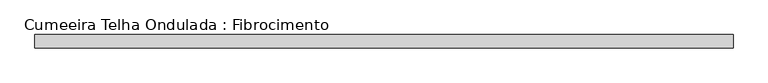
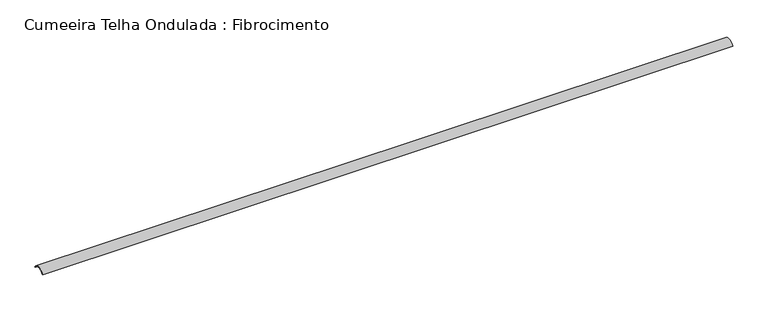
"""IFC4 building model written with IfcOpenShell, lengths in millimetres: beam geometry, Cumeeira Telha Ondulada : Fibrocimento."""

import ifcopenshell
import ifcopenshell.guid

model = None  # the IFC model being written
_history = None  # IfcOwnerHistory: only IFC2X3 demands one
_inside = {}  # id of a spatial element -> (the spatial element, [elements in it])
_under = {}  # id of a project, library or spatial element -> (it, [spatial elements below it])
_declared = {}  # id of a project -> (the project, [libraries it declares])
_typed = {}  # id of a type object -> (the type object, [elements of that type])
_made_of = {}  # id of a material, layer set ... -> (it, [elements and type objects made of it])


def new_model(schema):
    """Start an empty IFC model of exactly this schema.

    Asked for "IFC4X3", IfcOpenShell would pick the latest addendum, in which some entities
    have other attributes; the version numbers below select the first issue.
    IFC2X3 requires an IfcOwnerHistory on every rooted entity: one is made here for all.
    """
    global model, _history
    if schema == "IFC4X3":
        model = ifcopenshell.file(schema_version=(4, 3, 0, 0))
    else:
        model = ifcopenshell.file(schema=schema)
    _inside.clear()
    _under.clear()
    _declared.clear()
    _typed.clear()
    _made_of.clear()
    _history = None
    if model.schema == "IFC2X3":
        org = make("IfcOrganization", Name="unknown")
        user = make(
            "IfcPersonAndOrganization",
            ThePerson=make("IfcPerson", FamilyName="unknown"),
            TheOrganization=org,
        )
        app = make(
            "IfcApplication",
            ApplicationDeveloper=org,
            Version="unknown",
            ApplicationFullName="unknown",
            ApplicationIdentifier="unknown",
        )
        _history = make(
            "IfcOwnerHistory",
            OwningUser=user,
            OwningApplication=app,
            ChangeAction="ADDED",
            CreationDate=0,
        )
    return model


def make(cls, **values):
    """One entity of the class cls with the attributes given. An attribute that is None is left unset."""
    return model.create_entity(
        cls, **{name: value for name, value in values.items() if value is not None}
    )


def rooted(cls, **values):
    """An entity with a GlobalId (a new one), such as an element, a storey or a relation."""
    return make(cls, GlobalId=ifcopenshell.guid.new(), OwnerHistory=_history, **values)


def si_unit(unit_type, name, prefix=None):
    """IfcSIUnit, for example si_unit("LENGTHUNIT", "METRE", prefix="MILLI")."""
    return make("IfcSIUnit", UnitType=unit_type, Prefix=prefix, Name=name)


def assignment(units):
    """IfcUnitAssignment: the units of a project."""
    return None if units is None else make("IfcUnitAssignment", Units=units)


def point(xyz):
    """IfcCartesianPoint."""
    return None if xyz is None else make("IfcCartesianPoint", Coordinates=xyz)


def direction(xyz):
    """IfcDirection."""
    return None if xyz is None else make("IfcDirection", DirectionRatios=xyz)


def frame(location, z_axis=None, x_axis=None):
    """IfcAxis2Placement3D, a coordinate frame: its origin and axes. An axis left out is left unset."""
    return make(
        "IfcAxis2Placement3D",
        Location=point(location),
        Axis=direction(z_axis),
        RefDirection=direction(x_axis),
    )


def frame_2d(location, x_axis=None):
    """IfcAxis2Placement2D, a coordinate frame in the plane: its origin and x axis."""
    return make(
        "IfcAxis2Placement2D", Location=point(location), RefDirection=direction(x_axis)
    )


def origin():
    """The frame at (0, 0, 0) with its axes left unset."""
    return frame((0.0, 0.0, 0.0))


def place(relative_to, where):
    """IfcLocalPlacement: puts the frame where relative to a parent placement (None: the world)."""
    return make(
        "IfcLocalPlacement", PlacementRelTo=relative_to, RelativePlacement=where
    )


def context(
    kind, dimensions, precision=None, world=None, true_north=None, identifier=None
):
    """IfcGeometricRepresentationContext, for example the 3D "Model" context."""
    return make(
        "IfcGeometricRepresentationContext",
        ContextIdentifier=identifier,
        ContextType=kind,
        CoordinateSpaceDimension=dimensions,
        Precision=precision,
        WorldCoordinateSystem=world,
        TrueNorth=true_north,
    )


def project(units=None, contexts=None):
    """IfcProject with its units and contexts."""
    return rooted(
        "IfcProject",
        Name="project",
        RepresentationContexts=contexts,
        UnitsInContext=assignment(units),
    )


def spatial(cls, under=None, at=None, **own):
    """A site, building, storey or space (cls), placed at a placement, below another one or the project."""
    s = rooted(cls, ObjectPlacement=at, **own)
    if under is not None:
        _under.setdefault(under.id(), (under, []))[1].append(s)
    return s


def polyline(points):
    """IfcPolyline through the points."""
    return make("IfcPolyline", Points=[point(p) for p in points])


def circle_curve(where, radius):
    """IfcCircle in the frame where."""
    return make("IfcCircle", Position=where, Radius=radius)


def trimmed(basis, trim1, trim2, sense, master):
    """IfcTrimmedCurve: the piece of a basis curve between two trims."""
    return make(
        "IfcTrimmedCurve",
        BasisCurve=basis,
        Trim1=trim1,
        Trim2=trim2,
        SenseAgreement=sense,
        MasterRepresentation=master,
    )


def segment(curve, same_sense, transition):
    """IfcCompositeCurveSegment."""
    return make(
        "IfcCompositeCurveSegment",
        Transition=transition,
        SameSense=same_sense,
        ParentCurve=curve,
    )


def composite_curve(segments, self_intersect=None):
    """IfcCompositeCurve: segments joined end to end."""
    return make("IfcCompositeCurve", Segments=segments, SelfIntersect=self_intersect)


def outline(outer, holes=None, kind="AREA"):
    """IfcArbitraryClosedProfileDef: a profile drawn as a closed curve; with holes, ...WithVoids."""
    if holes is None:
        return make("IfcArbitraryClosedProfileDef", ProfileType=kind, OuterCurve=outer)
    return make(
        "IfcArbitraryProfileDefWithVoids",
        ProfileType=kind,
        OuterCurve=outer,
        InnerCurves=holes,
    )


def extrude(swept, where, along, depth):
    """IfcExtrudedAreaSolid: the profile swept, set in the frame where, extruded along a direction by depth."""
    return make(
        "IfcExtrudedAreaSolid",
        SweptArea=swept,
        Position=where,
        ExtrudedDirection=direction(along),
        Depth=depth,
    )


def shape(context_of_items, identifier, shape_type, items):
    """IfcShapeRepresentation: the items that make up one representation, for example the "Body"."""
    return make(
        "IfcShapeRepresentation",
        ContextOfItems=context_of_items,
        RepresentationIdentifier=identifier,
        RepresentationType=shape_type,
        Items=items,
    )


def source(mapping_origin, context_of_items, identifier, shape_type, items):
    """IfcRepresentationMap: a shape defined once, which mapped items show again and again."""
    return make(
        "IfcRepresentationMap",
        MappingOrigin=mapping_origin,
        MappedRepresentation=shape(context_of_items, identifier, shape_type, items),
    )


def transform(
    local_origin,
    x_axis=None,
    y_axis=None,
    z_axis=None,
    scale=None,
    scale2=None,
    scale3=None,
    uniform=True,
):
    """IfcCartesianTransformationOperator3D, or its non-uniform kind. x_axis, y_axis, z_axis: its Axis1, 2, 3."""
    if uniform:
        return make(
            "IfcCartesianTransformationOperator3D",
            Axis1=direction(x_axis),
            Axis2=direction(y_axis),
            LocalOrigin=point(local_origin),
            Scale=scale,
            Axis3=direction(z_axis),
        )
    return make(
        "IfcCartesianTransformationOperator3DnonUniform",
        Axis1=direction(x_axis),
        Axis2=direction(y_axis),
        LocalOrigin=point(local_origin),
        Scale=scale,
        Axis3=direction(z_axis),
        Scale2=scale2,
        Scale3=scale3,
    )


def mapped(mapping_source, mapping_target):
    """IfcMappedItem: shows the shape of a source again, moved by a transform."""
    return make(
        "IfcMappedItem", MappingSource=mapping_source, MappingTarget=mapping_target
    )


def made_of(thing, what):
    """Note that an element or type object is made of a material, layer set ...; save() writes the relation."""
    if what is not None:
        _made_of.setdefault(what.id(), (what, []))[1].append(thing)
    return thing


def element(
    cls,
    number,
    at=None,
    inside=None,
    cuts=None,
    type_object=None,
    material=None,
    context=None,
    identifier="Body",
    shape_type=None,
    held_by="IfcProductDefinitionShape",
    body=None,
    shapes=None,
    **own,
):
    """One element of the class cls, such as IfcWall. Its Tag is "e" and its number.

    at: its placement. inside: the storey or other place that contains it. cuts: it is an
    opening in that element (IfcRelVoidsElement). A single representation is given by context,
    identifier, shape_type and body (its items); several are given by shapes. held_by: the class
    of the entity that holds the representations. save() writes the other relations.
    """
    e = rooted(cls, Tag="e%d" % number, ObjectPlacement=at, **own)
    if body is not None:
        shapes = [shape(context, identifier, shape_type, body)]
    if shapes is not None:
        e.Representation = make(held_by, Representations=shapes)
    if inside is not None:
        _inside.setdefault(inside.id(), (inside, []))[1].append(e)
    if cuts is not None:
        rooted(
            "IfcRelVoidsElement", RelatingBuildingElement=cuts, RelatedOpeningElement=e
        )
    if type_object is not None:
        _typed.setdefault(type_object.id(), (type_object, []))[1].append(e)
    return made_of(e, material)


def aggregate(whole, parts):
    """IfcRelAggregates: a whole, such as a stair, and the parts it consists of."""
    return rooted("IfcRelAggregates", RelatingObject=whole, RelatedObjects=parts)


def save(model, path):
    """Write the relations noted so far, then the file.

    IfcRelAggregates (storeys below a building ...), IfcRelContainedInSpatialStructure (elements
    in a storey), IfcRelDefinesByType, IfcRelAssociatesMaterial and IfcRelDeclares: one each for
    every whole, place, type object, material and project.
    """
    for whole, parts in _under.values():
        aggregate(whole, parts)
    for where, things in _inside.values():
        rooted(
            "IfcRelContainedInSpatialStructure",
            RelatedElements=things,
            RelatingStructure=where,
        )
    for kind, things in _typed.values():
        rooted("IfcRelDefinesByType", RelatedObjects=things, RelatingType=kind)
    for what, things in _made_of.values():
        rooted("IfcRelAssociatesMaterial", RelatedObjects=things, RelatingMaterial=what)
    for by, libraries in _declared.values():
        rooted("IfcRelDeclares", RelatingContext=by, RelatedDefinitions=libraries)
    model.write(path)


def cumeeira_telha_ondulada_fibrocimento_e54732c7(model_context):
    return source(origin(), model_context, "Body", "SweptSolid", [
        extrude(outline(composite_curve([segment(polyline([(58.3970135, 42.4437972), (53.9055884, 40.2467307)]), True, "CONTINUOUS"), segment(trimmed(circle_curve(frame_2d((-1.6029865, 13.0936483)), 61.7939461), [point((53.9055884, 40.2467307))], [point((-57.1115615, 40.2467307))], True, "CARTESIAN"), True, "CONTINUOUS"), segment(polyline([(-57.1115615, 40.2467307), (-61.6029865, 42.4437972)]), True, "CONTINUOUS"), segment(trimmed(circle_curve(frame_2d((-1.6029865, 13.0936483)), 66.7939461), [point((-61.6029865, 42.4437972))], [point((58.3970135, 42.4437972))], False, "CARTESIAN"), True, "CONTINUOUS")], self_intersect=False)), frame((-3133.4781794, 0.0, 0.0), z_axis=(1.0, 0.0, 0.0), x_axis=(0.0, 1.0, 0.0)), (0.0, 0.0, 1.0), 6266.9563589),
    ])


if __name__ == "__main__":
    model = new_model("IFC4")
    model_context = context("Model", 3, world=origin())
    ifc_project = project(units=[si_unit("LENGTHUNIT", "METRE", prefix="MILLI")], contexts=[model_context])
    site = spatial("IfcSite", under=ifc_project)
    building = spatial("IfcBuilding", under=site)
    placement = place(None, origin())
    cumeeira_telha_ondulada_fibrocimento_shape = cumeeira_telha_ondulada_fibrocimento_e54732c7(model_context)
    element("IfcBeam", 1, ObjectType="Cumeeira Telha Ondulada : Fibrocimento", at=placement, inside=building, context=model_context, shape_type="MappedRepresentation", body=[
        mapped(cumeeira_telha_ondulada_fibrocimento_shape, transform((0.0, 0.0, 0.0), x_axis=(1.0, 0.0, 0.0), y_axis=(0.0, 1.0, 0.0), z_axis=(0.0, 0.0, 1.0))),
    ])
    save(model, "model.ifc")

# Revit data of these elements
# Type "Cumeeira Telha Ondulada : Fibrocimento"
#   Cost = 5
#   Length [instance default] = 1.524 m
#   b = 0.07 m
#   h = 0.16 m
#   Structural Material = .TELHA DE FIBROCIMENTO
#   Assembly Code = ""
# Element 1 (IfcBeam, "Cumeeira Telha Ondulada : Fibrocimento")
#   Materials on its faces: ".TELHA DE FIBROCIMENTO"
# Materials
#   ".TELHA DE FIBROCIMENTO": class "CC_TELHADO", colour RGB 77 77 76, transparency 0, Description = "TELHA ONDULADA FIBROCIMENTO", Cost = 0
